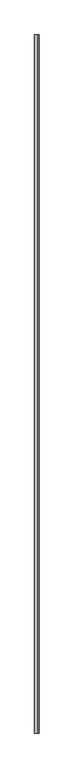
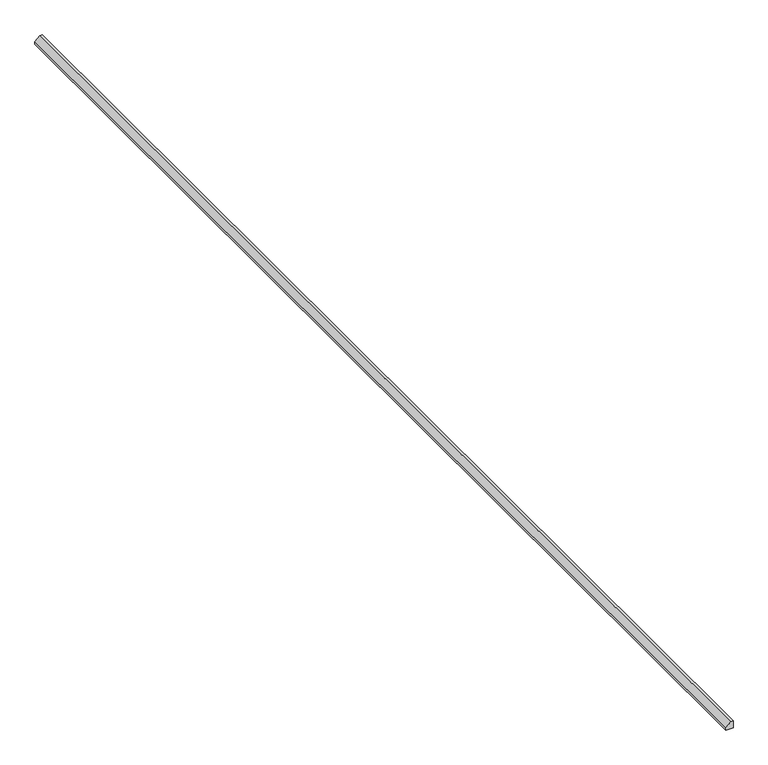
"""IFC4 building model written with IfcOpenShell, lengths in millimetres: proxy geometry, Stephan Brady6 : Stephan Brady."""

from ifc_helpers import new_model, si_unit, frame, origin, place, context, project, spatial, polyline, outline, extrude, source, transform, mapped, element, save


def generic_models_0edfd5c9(model_context):
    return source(origin(), model_context, "Body", "SweptSolid", [
        extrude(outline(polyline([(3226.308, -1731.9268771), (3226.308, -1738.2768771), (3213.608, -1750.9768771), (3207.258, -1750.9768771), (3207.258, -1731.9268771), (3226.308, -1731.9268771)])), frame((0.0, -3264.0948735, 0.0), z_axis=(0.0, 1.0, 0.0), x_axis=(0.0, 0.0, 1.0)), (0.0, 0.0, 1.0), 3176.5953427),
    ])


if __name__ == "__main__":
    model = new_model("IFC4")
    model_context = context("Model", 3, world=origin())
    ifc_project = project(units=[si_unit("LENGTHUNIT", "METRE", prefix="MILLI")], contexts=[model_context])
    site = spatial("IfcSite", under=ifc_project)
    building = spatial("IfcBuilding", under=site)
    placement = place(None, origin())
    generic_models_shape = generic_models_0edfd5c9(model_context)
    element("IfcBuildingElementProxy", 1, Name="Stephan Brady6 : Stephan Brady", ObjectType="Stephan Brady6 : Stephan Brady", at=placement, inside=building, context=model_context, shape_type="MappedRepresentation", body=[
        mapped(generic_models_shape, transform((0.0, 0.0, 0.0), x_axis=(1.0, 0.0, 0.0), y_axis=(0.0, 1.0, 0.0), z_axis=(0.0, 0.0, 1.0))),
    ])
    save(model, "model.ifc")

# Revit data of these elements
# Element 1 (IfcBuildingElementProxy, "Stephan Brady6 : Stephan Brady")
#   Materials on its faces: "Aluminum"
# Materials
#   "Aluminum": class "Metal", colour RGB 247 247 247, transparency 0, Description = "Aluminum 6061", Cost = 0
